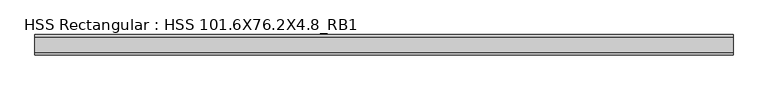
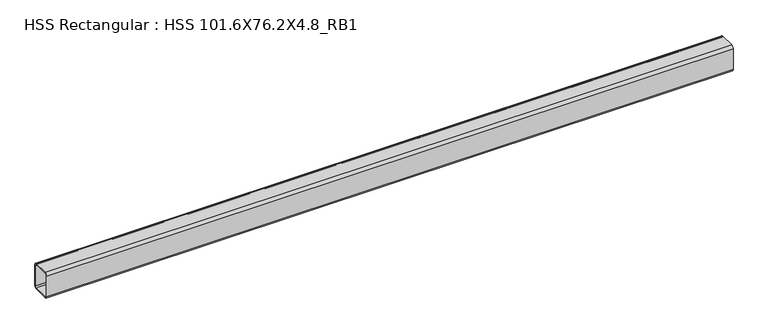
"""IFC4 building model written with IfcOpenShell, lengths in millimetres: beam geometry, HSS Rectangular : HSS 101.6X76.2X4.8_RB1."""

from ifc_helpers import new_model, si_unit, point, frame, frame_2d, origin, place, context, project, spatial, polyline, circle_curve, trimmed, segment, composite_curve, outline, extrude, source, transform, mapped, element, save


def hss_rectangular_hss_101_6x76_2x4_8_rb1_d3b57e1d(model_context):
    return source(origin(), model_context, "Body", "SweptSolid", [
        extrude(outline(composite_curve([segment(polyline([(38.1, 41.275), (38.1, -41.275)]), True, "CONTINUOUS"), segment(trimmed(circle_curve(frame_2d((28.575, -41.275)), 9.525), [point((38.1, -41.275))], [point((28.575, -50.8))], False, "CARTESIAN"), True, "CONTINUOUS"), segment(polyline([(28.575, -50.8), (-28.575, -50.8)]), True, "CONTINUOUS"), segment(trimmed(circle_curve(frame_2d((-28.575, -41.275)), 9.525), [point((-28.575, -50.8))], [point((-38.1, -41.275))], False, "CARTESIAN"), True, "CONTINUOUS"), segment(polyline([(-38.1, -41.275), (-38.1, 41.275)]), True, "CONTINUOUS"), segment(trimmed(circle_curve(frame_2d((-28.575, 41.275)), 9.525), [point((-38.1, 41.275))], [point((-28.575, 50.8))], False, "CARTESIAN"), True, "CONTINUOUS"), segment(polyline([(-28.575, 50.8), (28.575, 50.8)]), True, "CONTINUOUS"), segment(trimmed(circle_curve(frame_2d((28.575, 41.275)), 9.525), [point((28.575, 50.8))], [point((38.1, 41.275))], False, "CARTESIAN"), True, "CONTINUOUS")], self_intersect=False), holes=[composite_curve([segment(trimmed(circle_curve(frame_2d((-28.575, 41.275)), 4.7625), [point((-28.575, 46.0375))], [point((-33.3375, 41.275))], True, "CARTESIAN"), True, "CONTINUOUS"), segment(polyline([(-33.3375, 41.275), (-33.3375, -41.275)]), True, "CONTINUOUS"), segment(trimmed(circle_curve(frame_2d((-28.575, -41.275)), 4.7625), [point((-33.3375, -41.275))], [point((-28.575, -46.0375))], True, "CARTESIAN"), True, "CONTINUOUS"), segment(polyline([(-28.575, -46.0375), (28.575, -46.0375)]), True, "CONTINUOUS"), segment(trimmed(circle_curve(frame_2d((28.575, -41.275)), 4.7625), [point((28.575, -46.0375))], [point((33.3375, -41.275))], True, "CARTESIAN"), True, "CONTINUOUS"), segment(polyline([(33.3375, -41.275), (33.3375, 41.275)]), True, "CONTINUOUS"), segment(trimmed(circle_curve(frame_2d((28.575, 41.275)), 4.7625), [point((33.3375, 41.275))], [point((28.575, 46.0375))], True, "CARTESIAN"), True, "CONTINUOUS"), segment(polyline([(28.575, 46.0375), (-28.575, 46.0375)]), True, "CONTINUOUS")], self_intersect=False)]), frame((-1331.0900009, 0.0, 0.0), z_axis=(1.0, 0.0, 0.0), x_axis=(0.0, 1.0, 0.0)), (0.0, 0.0, 1.0), 2611.7000012),
    ])


if __name__ == "__main__":
    model = new_model("IFC4")
    model_context = context("Model", 3, world=origin())
    ifc_project = project(units=[si_unit("LENGTHUNIT", "METRE", prefix="MILLI")], contexts=[model_context])
    site = spatial("IfcSite", under=ifc_project)
    building = spatial("IfcBuilding", under=site)
    placement = place(None, origin())
    hss_rectangular_hss_101_6x76_2x4_8_rb1_shape = hss_rectangular_hss_101_6x76_2x4_8_rb1_d3b57e1d(model_context)
    element("IfcBeam", 1, ObjectType="HSS Rectangular : HSS 101.6X76.2X4.8_RB1", at=placement, inside=building, context=model_context, shape_type="MappedRepresentation", body=[
        mapped(hss_rectangular_hss_101_6x76_2x4_8_rb1_shape, transform((0.0, 0.0, 0.0), x_axis=(1.0, 0.0, 0.0), y_axis=(0.0, 1.0, 0.0), z_axis=(0.0, 0.0, 1.0))),
    ])
    save(model, "model.ifc")

# Revit data of these elements
# Type "HSS Rectangular : HSS 101.6X76.2X4.8_RB1"
#   Section Name Key = "HSS 4X3X3/16"
#   Assembly Code = "B10"
#   Width = 7.62 cm
#   Wall Nominal Thickness = 0.4763 cm
#   Wall Design Thickness = 0.442 cm
#   Torsional Moment of Inertia = 260.561 cm⁴
#   Torsional Modulus = 61.2876 cm³
#   Section Area = 14.4516 cm²
#   Plastic Modulus weak axis = 40.3122 cm³
#   Plastic Modulus strong axis = 49.1612 cm³
#   Perimeter = 0.881482 m²/m
#   Outer Fillet = 0.9525 cm
#   Nominal Weight = 12.1285 kgf/m
#   Moment of Inertia weak axis = 131.529 cm⁴
#   Moment of Inertia strong axis = 205.202 cm⁴
#   Inner Fillet = 0.4763 cm
#   Height = 10.16 cm
#   Elastic Modulus weak axis = 34.4128 cm³
#   Elastic Modulus strong axis = 40.476 cm³
#   Centroid Vertical = 5.08 cm
#   Centroid Horizontal = 3.81 cm
#   Length [instance default] = 1524 mm
#   Structural Material [instance default] = Steel ASTM A500, Grade B, Rectangular and Square
#   Principal Axes Angle = 0
# Element 1 (IfcBeam, "HSS Rectangular : HSS 101.6X76.2X4.8_RB1")
#   Structural Material = Steel ASTM A992
#   Materials on its faces: "Steel ASTM A992"
# Materials
#   "Steel ASTM A500, Grade B, Rectangular and Square": class "Metal", colour RGB 199 199 199, transparency 0, Description = "Carbon steel", Cost = 0
#   "Steel ASTM A992": class "Metal", colour RGB 199 199 199, transparency 0, Description = "Structural steel 50ksi", Cost = 0
